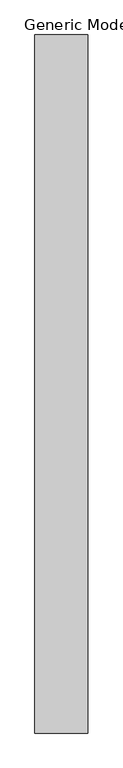
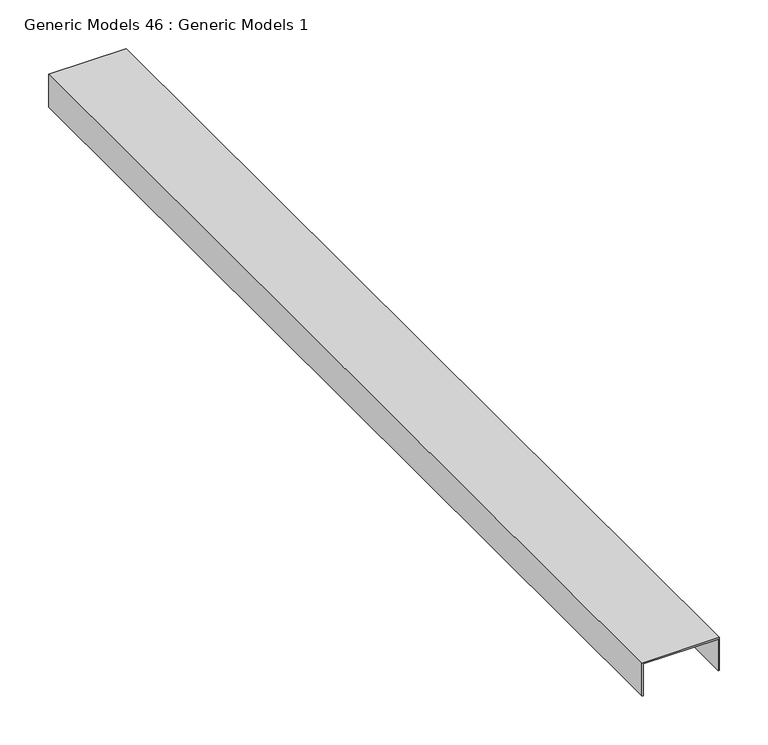
"""IFC4 building model written with IfcOpenShell, lengths in millimetres: proxy geometry, Generic Models 46 : Generic Models 1."""

from ifc_helpers import new_model, si_unit, frame, origin, place, context, project, spatial, polyline, outline, extrude, source, transform, mapped, element, save


def generic_models_46_generic_models_1_467ce512(model_context):
    return source(origin(), model_context, "Body", "SweptSolid", [
        extrude(outline(polyline([(393.2679367, 50793.65), (351.9929367, 50793.65), (351.9929367, 50795.2375), (391.6804367, 50795.2375), (391.6804367, 50884.1375), (351.9929367, 50884.1375), (351.9929367, 50885.725), (393.2679367, 50885.725), (393.2679367, 50793.65)])), frame((0.0, 0.0, 0.0), z_axis=(0.0, 1.0, 0.0), x_axis=(0.0, 0.0, 1.0)), (0.0, 0.0, 1.0), 1219.2),
    ])


if __name__ == "__main__":
    model = new_model("IFC4")
    model_context = context("Model", 3, world=origin())
    ifc_project = project(units=[si_unit("LENGTHUNIT", "METRE", prefix="MILLI")], contexts=[model_context])
    site = spatial("IfcSite", under=ifc_project)
    building = spatial("IfcBuilding", under=site)
    placement = place(None, origin())
    generic_models_46_generic_models_1_shape = generic_models_46_generic_models_1_467ce512(model_context)
    element("IfcBuildingElementProxy", 1, Name="Generic Models 46 : Generic Models 1", ObjectType="Generic Models 46 : Generic Models 1", at=placement, inside=building, context=model_context, shape_type="MappedRepresentation", body=[
        mapped(generic_models_46_generic_models_1_shape, transform((0.0, 0.0, 0.0), x_axis=(1.0, 0.0, 0.0), y_axis=(0.0, 1.0, 0.0), z_axis=(0.0, 0.0, 1.0))),
    ])
    save(model, "model.ifc")

# Revit data of these elements
# Element 1 (IfcBuildingElementProxy, "Generic Models 46 : Generic Models 1")
#   Materials on its faces: "METAL RUNNER ANCHORED TO STRUCTURE"
# Materials
#   "METAL RUNNER ANCHORED TO STRUCTURE": class "Unassigned", colour RGB 210 209 208, transparency 0, Keynote = "M05121300.02", Cost = 0
